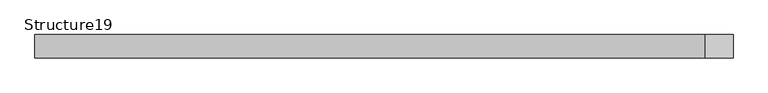
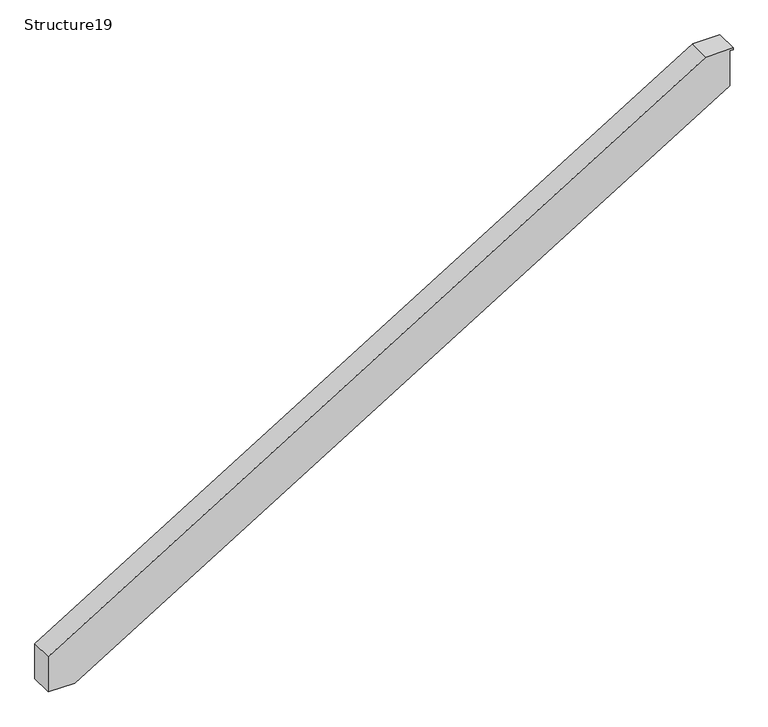
"""IFC4 building model written with IfcOpenShell, lengths in millimetres: proxy geometry, Structure19 : Structure668217140."""

from ifc_helpers import new_model, si_unit, origin, place, context, project, spatial, faceted_brep, source, transform, mapped, element, save


def structure19_2234788d(model_context):
    return source(origin(), model_context, "Body", "Brep", [
        faceted_brep([(4990.3637308, 1856.3038322, 36999.1950782), (4990.3637308, 1856.3038322, 36709.0959962), (5197.5264371, 1856.3038322, 36709.0959962), (10310.5384869, 1856.3038322, 39847.7170886), (10310.5384869, 1856.3038322, 40138.096), (10338.2140827, 1856.3038322, 40138.096), (10338.2140827, 1856.3038322, 40150.796), (10124.4233335, 1856.3038322, 40150.796), (4990.3637308, 2034.1038322, 36999.1950782), (10124.4233335, 2034.1038322, 40150.796), (10338.2140827, 2034.1038322, 40150.796), (10338.2140827, 2034.1038322, 40138.096), (10287.3140827, 2034.1038322, 40138.096), (10287.3140827, 2034.1038322, 39848.3626708), (10310.5384869, 2034.1038322, 39862.6189652), (10310.5384869, 2034.1038322, 39847.7170886), (5197.5264371, 2034.1038322, 36709.0959962), (4990.3637308, 2034.1038322, 36709.0959962), (5003.0637308, 2034.1038322, 36721.7959962), (5193.939441, 2034.1038322, 36721.7959962), (5214.6285434, 2034.1038322, 36734.4959962), (5003.0637308, 2034.1038322, 36734.4959962), (4990.3637308, 1869.0038322, 36709.0959962), (5197.5264371, 1869.0038322, 36709.0959962), (10124.4233335, 2021.4038322, 40150.796), (10124.4233335, 1869.0038322, 40150.796), (4990.3637308, 2021.4038322, 36999.1950782), (4990.3637308, 1869.0038322, 36999.1950782), (5003.0637308, 2021.4038322, 36992.0891638), (10128.0103876, 2021.4038322, 40138.096), (10128.0103876, 1869.0038322, 40138.096), (5003.0637308, 1869.0038322, 36992.0891638), (10310.5384869, 1869.0038322, 40138.096), (10287.3140827, 2021.4038322, 40138.096), (5193.939441, 1869.0038322, 36721.7959962), (10310.5384869, 1869.0038322, 39862.6189652), (10287.3140827, 2021.4038322, 39848.3626708), (5214.6285434, 2021.4038322, 36734.4959962), (5003.0637308, 1869.0038322, 36721.7959962), (5003.0637308, 2021.4038322, 36734.4959962)], [[[0, 1, 2, 3, 4, 5, 6, 7]], [[8, 9, 10, 11, 12, 13, 14, 15, 16, 17], [18, 19, 20, 21]], [[2, 1, 22, 17, 16, 23]], [[15, 3, 2, 23, 16]], [[7, 6, 10, 9, 24, 25]], [[0, 7, 25, 24, 9, 8, 26, 27]], [[28, 29, 30, 31]], [[11, 5, 4, 32, 30, 29, 33, 12]], [[20, 19, 34, 35, 14, 13, 36, 37]], [[19, 18, 38, 34]], [[39, 37, 36, 33, 29, 28]], [[32, 35, 34, 38, 31, 30]], [[1, 0, 27, 26, 8, 17, 22]], [[18, 21, 39, 28, 31, 38]], [[13, 12, 33, 36]], [[4, 3, 15, 14, 35, 32]], [[6, 5, 11, 10]], [[21, 20, 37, 39]]]),
    ])


if __name__ == "__main__":
    model = new_model("IFC4")
    model_context = context("Model", 3, world=origin())
    ifc_project = project(units=[si_unit("LENGTHUNIT", "METRE", prefix="MILLI")], contexts=[model_context])
    site = spatial("IfcSite", under=ifc_project)
    building = spatial("IfcBuilding", under=site)
    placement = place(None, origin())
    structure19_shape = structure19_2234788d(model_context)
    element("IfcBuildingElementProxy", 1, Name="Structure19 : Structure668217140", ObjectType="Structure19 : Structure668217140", at=placement, inside=building, context=model_context, shape_type="MappedRepresentation", body=[
        mapped(structure19_shape, transform((0.0, 0.0, 0.0), x_axis=(1.0, 0.0, 0.0), y_axis=(0.0, 1.0, 0.0), z_axis=(0.0, 0.0, 1.0))),
    ])
    save(model, "model.ifc")

# Revit data of these elements
# Type "Structure19 : Structure668217140"
#   NameOverride = "Structure668217140"
# Element 1 (IfcBuildingElementProxy, "Structure19 : Structure668217140")
#   Materials on its faces: "STEEL TUBE STRINGER - METALIZED AND PAINTED - COLOR PER ARCHITECT"
# Materials
#   "STEEL TUBE STRINGER - METALIZED AND PAINTED - COLOR PER ARCHITECT": class "Unassigned", colour RGB 128 128 128, transparency 0, Cost = 0
